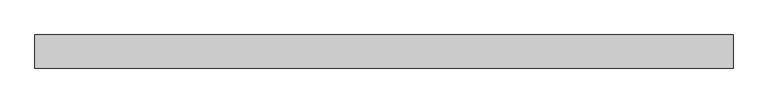
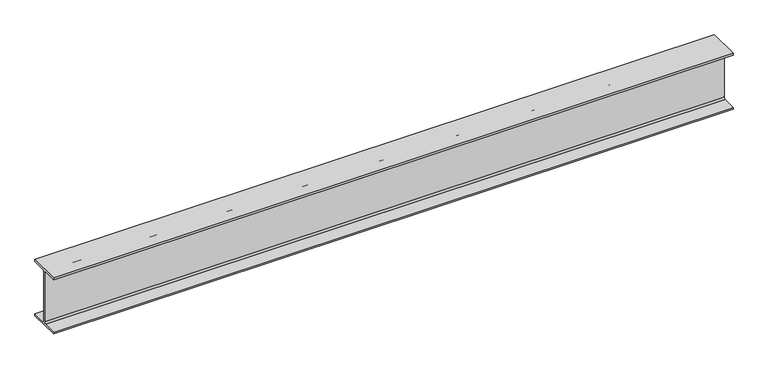
"""IFC4 building model written with IfcOpenShell, lengths in millimetres: beam geometry, Old_Steel Beam_H-KSD3502 : H_SB_ASB_H-200×200x8x12."""

import ifcopenshell
import ifcopenshell.guid

model = None  # the IFC model being written
_history = None  # IfcOwnerHistory: only IFC2X3 demands one
_inside = {}  # id of a spatial element -> (the spatial element, [elements in it])
_under = {}  # id of a project, library or spatial element -> (it, [spatial elements below it])
_declared = {}  # id of a project -> (the project, [libraries it declares])
_typed = {}  # id of a type object -> (the type object, [elements of that type])
_made_of = {}  # id of a material, layer set ... -> (it, [elements and type objects made of it])


def new_model(schema):
    """Start an empty IFC model of exactly this schema.

    Asked for "IFC4X3", IfcOpenShell would pick the latest addendum, in which some entities
    have other attributes; the version numbers below select the first issue.
    IFC2X3 requires an IfcOwnerHistory on every rooted entity: one is made here for all.
    """
    global model, _history
    if schema == "IFC4X3":
        model = ifcopenshell.file(schema_version=(4, 3, 0, 0))
    else:
        model = ifcopenshell.file(schema=schema)
    _inside.clear()
    _under.clear()
    _declared.clear()
    _typed.clear()
    _made_of.clear()
    _history = None
    if model.schema == "IFC2X3":
        org = make("IfcOrganization", Name="unknown")
        user = make(
            "IfcPersonAndOrganization",
            ThePerson=make("IfcPerson", FamilyName="unknown"),
            TheOrganization=org,
        )
        app = make(
            "IfcApplication",
            ApplicationDeveloper=org,
            Version="unknown",
            ApplicationFullName="unknown",
            ApplicationIdentifier="unknown",
        )
        _history = make(
            "IfcOwnerHistory",
            OwningUser=user,
            OwningApplication=app,
            ChangeAction="ADDED",
            CreationDate=0,
        )
    return model


def make(cls, **values):
    """One entity of the class cls with the attributes given. An attribute that is None is left unset."""
    return model.create_entity(
        cls, **{name: value for name, value in values.items() if value is not None}
    )


def rooted(cls, **values):
    """An entity with a GlobalId (a new one), such as an element, a storey or a relation."""
    return make(cls, GlobalId=ifcopenshell.guid.new(), OwnerHistory=_history, **values)


def si_unit(unit_type, name, prefix=None):
    """IfcSIUnit, for example si_unit("LENGTHUNIT", "METRE", prefix="MILLI")."""
    return make("IfcSIUnit", UnitType=unit_type, Prefix=prefix, Name=name)


def assignment(units):
    """IfcUnitAssignment: the units of a project."""
    return None if units is None else make("IfcUnitAssignment", Units=units)


def point(xyz):
    """IfcCartesianPoint."""
    return None if xyz is None else make("IfcCartesianPoint", Coordinates=xyz)


def direction(xyz):
    """IfcDirection."""
    return None if xyz is None else make("IfcDirection", DirectionRatios=xyz)


def frame(location, z_axis=None, x_axis=None):
    """IfcAxis2Placement3D, a coordinate frame: its origin and axes. An axis left out is left unset."""
    return make(
        "IfcAxis2Placement3D",
        Location=point(location),
        Axis=direction(z_axis),
        RefDirection=direction(x_axis),
    )


def frame_2d(location, x_axis=None):
    """IfcAxis2Placement2D, a coordinate frame in the plane: its origin and x axis."""
    return make(
        "IfcAxis2Placement2D", Location=point(location), RefDirection=direction(x_axis)
    )


def origin():
    """The frame at (0, 0, 0) with its axes left unset."""
    return frame((0.0, 0.0, 0.0))


def place(relative_to, where):
    """IfcLocalPlacement: puts the frame where relative to a parent placement (None: the world)."""
    return make(
        "IfcLocalPlacement", PlacementRelTo=relative_to, RelativePlacement=where
    )


def context(
    kind, dimensions, precision=None, world=None, true_north=None, identifier=None
):
    """IfcGeometricRepresentationContext, for example the 3D "Model" context."""
    return make(
        "IfcGeometricRepresentationContext",
        ContextIdentifier=identifier,
        ContextType=kind,
        CoordinateSpaceDimension=dimensions,
        Precision=precision,
        WorldCoordinateSystem=world,
        TrueNorth=true_north,
    )


def project(units=None, contexts=None):
    """IfcProject with its units and contexts."""
    return rooted(
        "IfcProject",
        Name="project",
        RepresentationContexts=contexts,
        UnitsInContext=assignment(units),
    )


def spatial(cls, under=None, at=None, **own):
    """A site, building, storey or space (cls), placed at a placement, below another one or the project."""
    s = rooted(cls, ObjectPlacement=at, **own)
    if under is not None:
        _under.setdefault(under.id(), (under, []))[1].append(s)
    return s


def polyline(points):
    """IfcPolyline through the points."""
    return make("IfcPolyline", Points=[point(p) for p in points])


def circle_curve(where, radius):
    """IfcCircle in the frame where."""
    return make("IfcCircle", Position=where, Radius=radius)


def trimmed(basis, trim1, trim2, sense, master):
    """IfcTrimmedCurve: the piece of a basis curve between two trims."""
    return make(
        "IfcTrimmedCurve",
        BasisCurve=basis,
        Trim1=trim1,
        Trim2=trim2,
        SenseAgreement=sense,
        MasterRepresentation=master,
    )


def segment(curve, same_sense, transition):
    """IfcCompositeCurveSegment."""
    return make(
        "IfcCompositeCurveSegment",
        Transition=transition,
        SameSense=same_sense,
        ParentCurve=curve,
    )


def composite_curve(segments, self_intersect=None):
    """IfcCompositeCurve: segments joined end to end."""
    return make("IfcCompositeCurve", Segments=segments, SelfIntersect=self_intersect)


def outline(outer, holes=None, kind="AREA"):
    """IfcArbitraryClosedProfileDef: a profile drawn as a closed curve; with holes, ...WithVoids."""
    if holes is None:
        return make("IfcArbitraryClosedProfileDef", ProfileType=kind, OuterCurve=outer)
    return make(
        "IfcArbitraryProfileDefWithVoids",
        ProfileType=kind,
        OuterCurve=outer,
        InnerCurves=holes,
    )


def extrude(swept, where, along, depth):
    """IfcExtrudedAreaSolid: the profile swept, set in the frame where, extruded along a direction by depth."""
    return make(
        "IfcExtrudedAreaSolid",
        SweptArea=swept,
        Position=where,
        ExtrudedDirection=direction(along),
        Depth=depth,
    )


def shape(context_of_items, identifier, shape_type, items):
    """IfcShapeRepresentation: the items that make up one representation, for example the "Body"."""
    return make(
        "IfcShapeRepresentation",
        ContextOfItems=context_of_items,
        RepresentationIdentifier=identifier,
        RepresentationType=shape_type,
        Items=items,
    )


def source(mapping_origin, context_of_items, identifier, shape_type, items):
    """IfcRepresentationMap: a shape defined once, which mapped items show again and again."""
    return make(
        "IfcRepresentationMap",
        MappingOrigin=mapping_origin,
        MappedRepresentation=shape(context_of_items, identifier, shape_type, items),
    )


def transform(
    local_origin,
    x_axis=None,
    y_axis=None,
    z_axis=None,
    scale=None,
    scale2=None,
    scale3=None,
    uniform=True,
):
    """IfcCartesianTransformationOperator3D, or its non-uniform kind. x_axis, y_axis, z_axis: its Axis1, 2, 3."""
    if uniform:
        return make(
            "IfcCartesianTransformationOperator3D",
            Axis1=direction(x_axis),
            Axis2=direction(y_axis),
            LocalOrigin=point(local_origin),
            Scale=scale,
            Axis3=direction(z_axis),
        )
    return make(
        "IfcCartesianTransformationOperator3DnonUniform",
        Axis1=direction(x_axis),
        Axis2=direction(y_axis),
        LocalOrigin=point(local_origin),
        Scale=scale,
        Axis3=direction(z_axis),
        Scale2=scale2,
        Scale3=scale3,
    )


def mapped(mapping_source, mapping_target):
    """IfcMappedItem: shows the shape of a source again, moved by a transform."""
    return make(
        "IfcMappedItem", MappingSource=mapping_source, MappingTarget=mapping_target
    )


def made_of(thing, what):
    """Note that an element or type object is made of a material, layer set ...; save() writes the relation."""
    if what is not None:
        _made_of.setdefault(what.id(), (what, []))[1].append(thing)
    return thing


def element(
    cls,
    number,
    at=None,
    inside=None,
    cuts=None,
    type_object=None,
    material=None,
    context=None,
    identifier="Body",
    shape_type=None,
    held_by="IfcProductDefinitionShape",
    body=None,
    shapes=None,
    **own,
):
    """One element of the class cls, such as IfcWall. Its Tag is "e" and its number.

    at: its placement. inside: the storey or other place that contains it. cuts: it is an
    opening in that element (IfcRelVoidsElement). A single representation is given by context,
    identifier, shape_type and body (its items); several are given by shapes. held_by: the class
    of the entity that holds the representations. save() writes the other relations.
    """
    e = rooted(cls, Tag="e%d" % number, ObjectPlacement=at, **own)
    if body is not None:
        shapes = [shape(context, identifier, shape_type, body)]
    if shapes is not None:
        e.Representation = make(held_by, Representations=shapes)
    if inside is not None:
        _inside.setdefault(inside.id(), (inside, []))[1].append(e)
    if cuts is not None:
        rooted(
            "IfcRelVoidsElement", RelatingBuildingElement=cuts, RelatedOpeningElement=e
        )
    if type_object is not None:
        _typed.setdefault(type_object.id(), (type_object, []))[1].append(e)
    return made_of(e, material)


def aggregate(whole, parts):
    """IfcRelAggregates: a whole, such as a stair, and the parts it consists of."""
    return rooted("IfcRelAggregates", RelatingObject=whole, RelatedObjects=parts)


def save(model, path):
    """Write the relations noted so far, then the file.

    IfcRelAggregates (storeys below a building ...), IfcRelContainedInSpatialStructure (elements
    in a storey), IfcRelDefinesByType, IfcRelAssociatesMaterial and IfcRelDeclares: one each for
    every whole, place, type object, material and project.
    """
    for whole, parts in _under.values():
        aggregate(whole, parts)
    for where, things in _inside.values():
        rooted(
            "IfcRelContainedInSpatialStructure",
            RelatedElements=things,
            RelatingStructure=where,
        )
    for kind, things in _typed.values():
        rooted("IfcRelDefinesByType", RelatedObjects=things, RelatingType=kind)
    for what, things in _made_of.values():
        rooted("IfcRelAssociatesMaterial", RelatedObjects=things, RelatingMaterial=what)
    for by, libraries in _declared.values():
        rooted("IfcRelDeclares", RelatingContext=by, RelatedDefinitions=libraries)
    model.write(path)


def beam_ba096bdf(model_context):
    return source(origin(), model_context, "Body", "SweptSolid", [
        extrude(outline(composite_curve([segment(polyline([(-82.5, -141.5), (-11.9, -141.5)]), True, "CONTINUOUS"), segment(trimmed(circle_curve(frame_2d((-11.9, -132.6)), 8.9), [point((-11.9, -141.5))], [point((-3.0, -132.6))], True, "CARTESIAN"), True, "CONTINUOUS"), segment(polyline([(-3.0, -132.6), (-3.0, 132.6)]), True, "CONTINUOUS"), segment(trimmed(circle_curve(frame_2d((-11.9, 132.6)), 8.9), [point((-3.0, 132.6))], [point((-11.9, 141.5))], True, "CARTESIAN"), True, "CONTINUOUS"), segment(polyline([(-11.9, 141.5), (-82.5, 141.5), (-82.5, 151.7), (82.5, 151.7), (82.5, 141.5), (11.9, 141.5)]), True, "CONTINUOUS"), segment(trimmed(circle_curve(frame_2d((11.9, 132.6)), 8.9), [point((11.9, 141.5))], [point((3.0, 132.6))], True, "CARTESIAN"), True, "CONTINUOUS"), segment(polyline([(3.0, 132.6), (3.0, -132.6)]), True, "CONTINUOUS"), segment(trimmed(circle_curve(frame_2d((11.9, -132.6)), 8.9), [point((3.0, -132.6))], [point((11.9, -141.5))], True, "CARTESIAN"), True, "CONTINUOUS"), segment(polyline([(11.9, -141.5), (82.5, -141.5), (82.5, -151.7), (-82.5, -151.7), (-82.5, -141.5)]), True, "CONTINUOUS")], self_intersect=False)), frame((-1756.1912669, 0.0, 0.0), z_axis=(1.0, 0.0, 0.0), x_axis=(0.0, 1.0, 0.0)), (0.0, 0.0, 1.0), 3479.0025034),
    ])


if __name__ == "__main__":
    model = new_model("IFC4")
    model_context = context("Model", 3, world=origin())
    ifc_project = project(units=[si_unit("LENGTHUNIT", "METRE", prefix="MILLI")], contexts=[model_context])
    site = spatial("IfcSite", under=ifc_project)
    building = spatial("IfcBuilding", under=site)
    placement = place(None, origin())
    beam_shape = beam_ba096bdf(model_context)
    element("IfcBeam", 1, ObjectType="Old_Steel Beam_H-KSD3502 : H_SB_ASB_H-200×200x8x12", at=placement, inside=building, context=model_context, shape_type="MappedRepresentation", body=[
        mapped(beam_shape, transform((0.0, 0.0, 0.0), x_axis=(1.0, 0.0, 0.0), y_axis=(0.0, 1.0, 0.0), z_axis=(0.0, 0.0, 1.0))),
    ])
    save(model, "model.ifc")

# Revit data of these elements
# Type "Old_Steel Beam_H-KSD3502 : H_SB_ASB_H-200×200x8x12"
#   Width = 20.0 cm
#   Web Thickness = 0.8 cm
#   Web Fillet = 1.3 cm
#   Warping Constant = 141376.0 cm⁶
#   Torsional Moment of Inertia = 26.2485 cm⁴
#   Torsional Modulus = 1.0 cm³
#   Section Area = 63.53 cm²
#   Plastic Modulus weak axis = 244.0 cm³
#   Plastic Modulus strong axis = 525.0 cm³
#   Perimeter = 1.16 m²/m
#   Nominal Weight = 49.90 kgf/m
#   Moment of Inertia weak axis = 1600.00 cm⁴
#   Moment of Inertia strong axis = 4720.00 cm⁴
#   Height = 20.0 cm
#   Flange Thickness = 1.2 cm
#   Elastic Modulus weak axis = 160.0 cm³
#   Elastic Modulus strong axis = 472.0 cm³
#   Centroid Vertical = 10.0 cm
#   Centroid Horizontal = 10.0 cm
#   Length [instance default] = 1.5240 m
#   Structural Material [instance default] = Steel, 45-345
#   Assembly Code = ""
# Element 1 (IfcBeam, "Old_Steel Beam_H-KSD3502 : H_SB_ASB_H-200×200x8x12")
#   Structural Material = none
# Materials
#   "Steel, 45-345": class "Metal", colour RGB 189 187 185, transparency 0, Description = "Steel 345 MPa", Cost = 0
